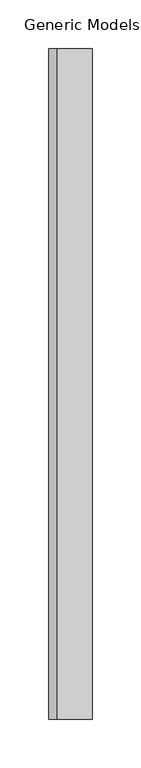
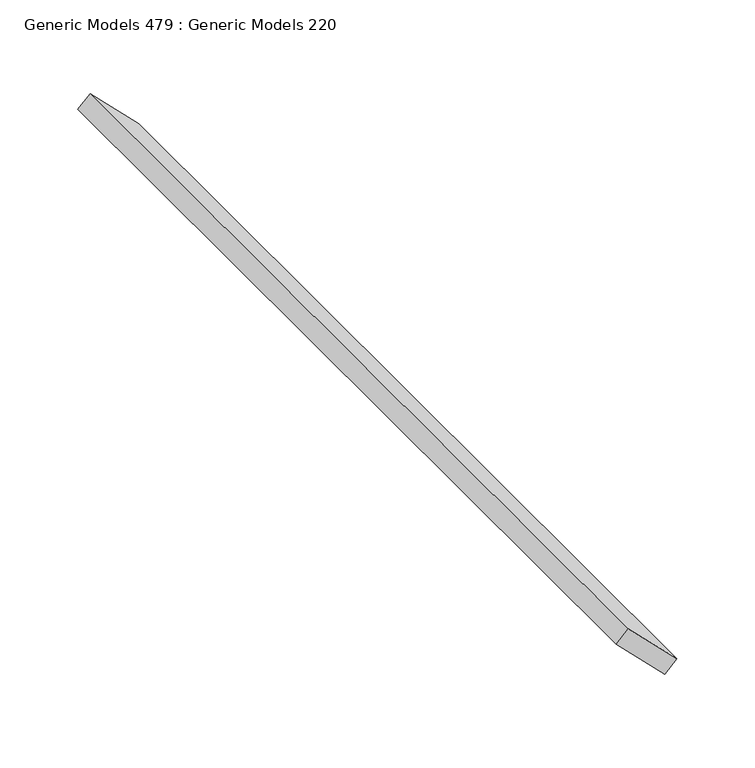
"""IFC4 building model written with IfcOpenShell, lengths in millimetres: proxy geometry, Generic Models 479 : Generic Models 220."""

from ifc_helpers import new_model, si_unit, frame, origin, place, context, project, spatial, polyline, outline, extrude, source, transform, mapped, element, save


def generic_models_479_generic_models_220_665a969d(model_context):
    return source(origin(), model_context, "Body", "SweptSolid", [
        extrude(outline(polyline([(0.0, -50.8), (0.0, 0.0), (690.8142348, 0.0), (690.8142348, -50.8), (0.0, -50.8)])), frame((-6899.085451, -4564.8872686, 127878.6762561), z_axis=(0.7071067811865582, 0.0, 0.7071067811865369), x_axis=(0.0, 1.0, 0.0)), (0.0, 0.0, 1.0), 12.7),
    ])


if __name__ == "__main__":
    model = new_model("IFC4")
    model_context = context("Model", 3, world=origin())
    ifc_project = project(units=[si_unit("LENGTHUNIT", "METRE", prefix="MILLI")], contexts=[model_context])
    site = spatial("IfcSite", under=ifc_project)
    building = spatial("IfcBuilding", under=site)
    placement = place(None, origin())
    generic_models_479_generic_models_220_shape = generic_models_479_generic_models_220_665a969d(model_context)
    element("IfcBuildingElementProxy", 1, Name="Generic Models 479 : Generic Models 220", ObjectType="Generic Models 479 : Generic Models 220", at=placement, inside=building, context=model_context, shape_type="MappedRepresentation", body=[
        mapped(generic_models_479_generic_models_220_shape, transform((0.0, 0.0, 0.0), x_axis=(1.0, 0.0, 0.0), y_axis=(0.0, 1.0, 0.0), z_axis=(0.0, 0.0, 1.0))),
    ])
    save(model, "model.ifc")

# Revit data of these elements
# Element 1 (IfcBuildingElementProxy, "Generic Models 479 : Generic Models 220")
#   Materials on its faces: "_WOOD TONE ALUMINUM EXTRUSION SLAT BY KNOTWOOD"
# Materials
#   "_WOOD TONE ALUMINUM EXTRUSION SLAT BY KNOTWOOD": class "Generic", colour RGB 177 130 114, transparency 0, Cost = 0
